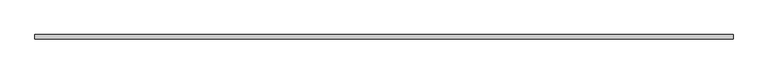
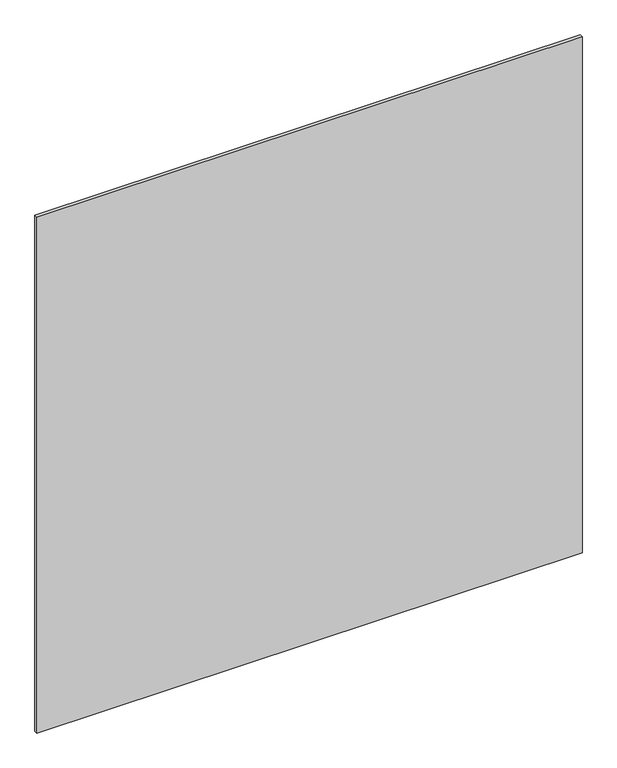
"""IFC4 building model written with IfcOpenShell, lengths in millimetres: proxy geometry, Panel1:Panel:306132:Panel:306132 : Panel1:Panel:306132:300355:Panel:306132:Panel:306132 : Panel1:Panel:306132:300355 : Panel1:Panel:306132:Panel:306132 : Panel1:Panel:306132:300355:2 : Panel1:Panel:306132:Panel:306132 : Panel1:Panel:306132:300355:Panel:306132:Panel:306132 : Panel1:Panel:306132:300355 : Panel1:Panel:306132:Panel:306132 : Panel1:Panel:306132:300355:300154."""

from ifc_helpers import new_model, si_unit, frame, origin, place, context, project, spatial, polyline, outline, extrude, source, transform, mapped, element, save


def generic_models_9809d970(model_context):
    return source(origin(), model_context, "Body", "SweptSolid", [
        extrude(outline(polyline([(593738.0867239, -579084.8288841), (593738.0867239, -579076.8913841), (594957.2867239, -579076.8913841), (594957.2867239, -579084.8288841), (593738.0867239, -579084.8288841)])), frame((0.0, 0.0, 2470.15), z_axis=(0.0, 0.0, 1.0), x_axis=(1.0, 0.0, 0.0)), (0.0, 0.0, 1.0), 1219.2),
    ])


if __name__ == "__main__":
    model = new_model("IFC4")
    model_context = context("Model", 3, world=origin())
    ifc_project = project(units=[si_unit("LENGTHUNIT", "METRE", prefix="MILLI")], contexts=[model_context])
    site = spatial("IfcSite", under=ifc_project)
    building = spatial("IfcBuilding", under=site)
    placement = place(None, origin())
    generic_models_shape = generic_models_9809d970(model_context)
    element("IfcBuildingElementProxy", 1, Name="Panel1:Panel:306132:Panel:306132 : Panel1:Panel:306132:300355:Panel:306132:Panel:306132 : Panel1:Panel:306132:300355 : Panel1:Panel:306132:Panel:306132 : Panel1:Panel:306132:300355:2 : Panel1:Panel:306132:Panel:306132 : Panel1:Panel:306132:300355:Panel:306132:Panel:306132 : Panel1:Panel:306132:300355 : Panel1:Panel:306132:Panel:306132 : Panel1:Panel:306132:300355:300154", ObjectType="Panel1:Panel:306132:Panel:306132 : Panel1:Panel:306132:300355:Panel:306132:Panel:306132 : Panel1:Panel:306132:300355 : Panel1:Panel:306132:Panel:306132 : Panel1:Panel:306132:300355:2 : Panel1:Panel:306132:Panel:306132 : Panel1:Panel:306132:300355:Panel:306132:Panel:306132 : Panel1:Panel:306132:300355 : Panel1:Panel:306132:Panel:306132 : Panel1:Panel:306132:300355:300154", at=placement, inside=building, context=model_context, shape_type="MappedRepresentation", body=[
        mapped(generic_models_shape, transform((0.0, 0.0, 0.0), x_axis=(1.0, 0.0, 0.0), y_axis=(0.0, 1.0, 0.0), z_axis=(0.0, 0.0, 1.0))),
    ])
    save(model, "model.ifc")

# Revit data of these elements
# Type "Panel1:Panel:306132:Panel:306132 : Panel1:Panel:306132:300355:Panel:306132:Panel:306132 : Panel1:Panel:306132:300355 : Panel1:Panel:306132:Panel:306132 : Panel1:Panel:306132:300355:2 : Panel1:Panel:306132:Panel:306132 : Panel1:Panel:306132:300355:Panel:306132:Panel:306132 : Panel1:Panel:306132:300355 : Panel1:Panel:306132:Panel:306132 : Panel1:Panel:306132:300355:300154"
#   NameOverride = "Panel1:Panel:306132:Panel:306132 : Panel1:Panel:306132:300355:Panel:306132:Panel:306132 : Panel1:Panel:306132:300355 : Panel1:Panel:306132:Panel:306132 : Panel1:Panel:306132:300355:300154"
#   ObjectTypeOverride = "Panel:306132:Panel:306132 : Panel1:Panel:306132:300355 : Panel1:Panel:306132:Panel:306132 : Panel1:Panel:306132:300355"
#   Reference = "Panel"
#   Tag = "300154"
# Element 1 (IfcBuildingElementProxy, "Panel1:Panel:306132:Panel:306132 : Panel1:Panel:306132:300355:Panel:306132:Panel:306132 : Panel1:Panel:306132:300355 : Panel1:Panel:306132:Panel:306132 : Panel1:Panel:306132:300355:2 : Panel1:Panel:306132:Panel:306132 : Panel1:Panel:306132:300355:Panel:306132:Panel:306132 : Panel1:Panel:306132:300355 : Panel1:Panel:306132:Panel:306132 : Panel1:Panel:306132:300355:300154")
#   Materials on its faces: "5/16\" PHENOLIC RESIN PANELS (CLASS A FLAME SPREAD) - EXPOSED FASTENERS"
# Materials
#   "5/16\" PHENOLIC RESIN PANELS (CLASS A FLAME SPREAD) - EXPOSED FASTENERS": class "Unassigned", colour RGB 64 64 64, transparency 0, Keynote = "M07420000.01", Cost = 0
